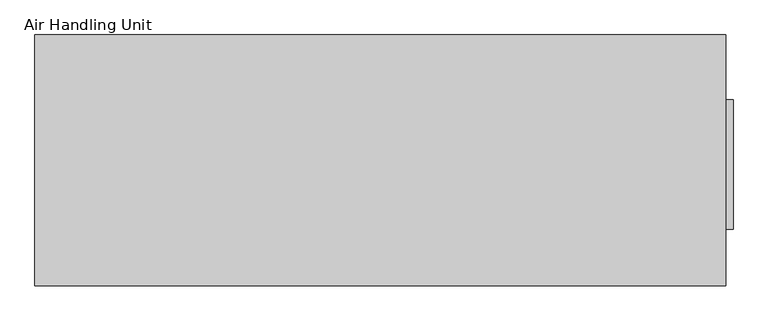
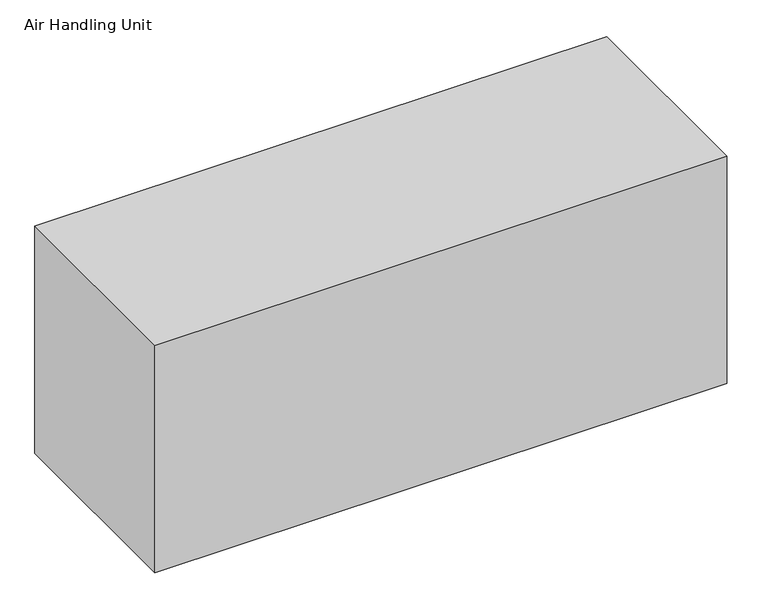
"""IFC4 building model written with IfcOpenShell, lengths in millimetres: proxy geometry, Air Handling Unit : 63300000 J."""

from ifc_helpers import new_model, si_unit, frame, origin, origin_with_axes, place, context, project, spatial, polyline, outline, extrude, source, transform, mapped, element, save


def air_handling_unit_7c967d2d(model_context):
    return source(origin(), model_context, "Body", "SweptSolid", [
        extrude(outline(polyline([(1486.0, 121.55), (1486.0, 400.95), (1501.875, 400.95), (1501.875, 121.55), (1486.0, 121.55)])), frame((0.0, 0.0, 187.5), z_axis=(0.0, 0.0, 1.0), x_axis=(1.0, 0.0, 0.0)), (0.0, 0.0, 1.0), 250.0),
        extrude(outline(polyline([(1486.0, 540.0), (1486.0, 0.0), (0.0, 0.0), (0.0, 540.0), (1486.0, 540.0)])), origin_with_axes(), (0.0, 0.0, 1.0), 625.0),
    ])


if __name__ == "__main__":
    model = new_model("IFC4")
    model_context = context("Model", 3, world=origin())
    ifc_project = project(units=[si_unit("LENGTHUNIT", "METRE", prefix="MILLI")], contexts=[model_context])
    site = spatial("IfcSite", under=ifc_project)
    building = spatial("IfcBuilding", under=site)
    placement = place(None, origin())
    air_handling_unit_shape = air_handling_unit_7c967d2d(model_context)
    element("IfcBuildingElementProxy", 1, Name="Air Handling Unit : 63300000 J", ObjectType="Air Handling Unit : 63300000 J", at=placement, inside=building, context=model_context, shape_type="MappedRepresentation", body=[
        mapped(air_handling_unit_shape, transform((0.0, 0.0, 0.0), x_axis=(1.0, 0.0, 0.0), y_axis=(0.0, 1.0, 0.0), z_axis=(0.0, 0.0, 1.0))),
    ])
    save(model, "model.ifc")

# Revit data of these elements
# Project information
#   Organization Name = "Prairie Sky Consulting"
#   Building Name = "Four Dormitory Project"
#   Author = "R.K."
#   COBie.CreatedBy = "info@mma.ie"
#   COBie.CreatedOn = "2017-07-21T10:57:54"
#   COBie.Facility.Category = "11-16 27 14 : Mixed-Gender Dormitory"
#   COBie.Facility.LinearUnits = "Millimeters"
#   COBie.Facility.AreaUnits = "Square Meters"
#   COBie.Facility.VolumeUnits = "Cubic Meters"
#   COBie.Facility.CurrencyUnit = "Dollar"
#   COBie.Facility.AreaMeasurement = "Revit Default Area Calculation Method"
#   COBie.Facility.Description = "One Four Dormitories Project Site on the E,Healey Site"
#   COBie.Facility.ProjectDescription = "A two Story luxury Dormitory"
#   COBie.Facility.SiteDescription = "Four Dormitories Project Site"
#   COBie.Facility.Phase = "60% Design Submission"
#   Classification.Facility.Description = "Mixed-Gender Dormitory"
#   Classification.Facility.Number = "11-16 27 14"
#   Project Issue Date = "Issue Date"
#   Project Status = "Final Issue"
#   Client Name = "Prairie Sky Consulting"
#   Project Address = "East Healy Street,\nChampaign,\nIllinois,\nUSA"
#   Project Name = "Four Dormitory Complex"
#   Project Number = "East Dormitory"
# Type "Air Handling Unit : 63300000 J"
#   Type Mark = "Air Handling Unit"
#   COBie.Type.CreatedBy = "info@mma.ie"
#   COBie.Type.CreatedOn = "2017-07-21T10:57:54"
#   COBie.Type.Name = "Air Handling Unit"
#   COBie.Type.Category = "23-33 25 00 : Air Handling Units"
#   COBie.Type.Description = "Air Handling Unit_63300000 J"
#   COBie.Type.AssetType = "Fixed"
#   COBie.Type.Manufacturer = ""
#   COBie.Type.ModelNumber = ""
#   Classification.OmniClass.23.Number = "23-33 25 00"
#   Classification.OmniClass.23.Description = "Air Handling Units"
#   Keynote = "23 06 70.13.A"
#   COBie.Type.ReplacementCost = 0
#   Width = 540 mm
#   Voltage = 230 V
#   External Static Pressure [instance default] = 0.498312 in-wg
#   Supply Airflow [instance default] = 1777.74 CFM
#   Return Airflow [instance default] = 1777.74 CFM
#   Length = 1486 mm
#   Height = 625 mm
#   Heating Capacity = 60665711 J
#   Dimension H = 791 mm
#   Dimension G = 695 mm
#   Dimension F = 300 mm
#   Dimension E = 300 mm
#   Dimension D = 250 mm
#   Dimension A = 450 mm
#   Cooling Capacity = 56445488 J
#   Condensate Radius = 10 mm
#   Condensate Diameter = 20 mm
#   Apparent Load = 1040 VA
#   AHU Supply Airflow [instance default] = 1777.74 CFM
#   AHU Return Airflow [instance default] = 1777.74 CFM
#   AHU Heating Capacity = 60665711 J
#   AHU Cooling Capacity = 56445488 J
#   AHU Apparant Load = 1040 VA
#   COBie.Type = yes
#   Poles = 1
#   Load Classification = Cooling
#   Default Elevation = 0
#   Assembly Code = ""
# Element 1 (IfcBuildingElementProxy, "Air Handling Unit : 63300000 J")
#   Supply Airflow = 0.0 CFM
#   Return Airflow = 1101.82 CFM
#   AHU Supply Airflow = 0.0 CFM
#   AHU Return Airflow = 1101.82 CFM
